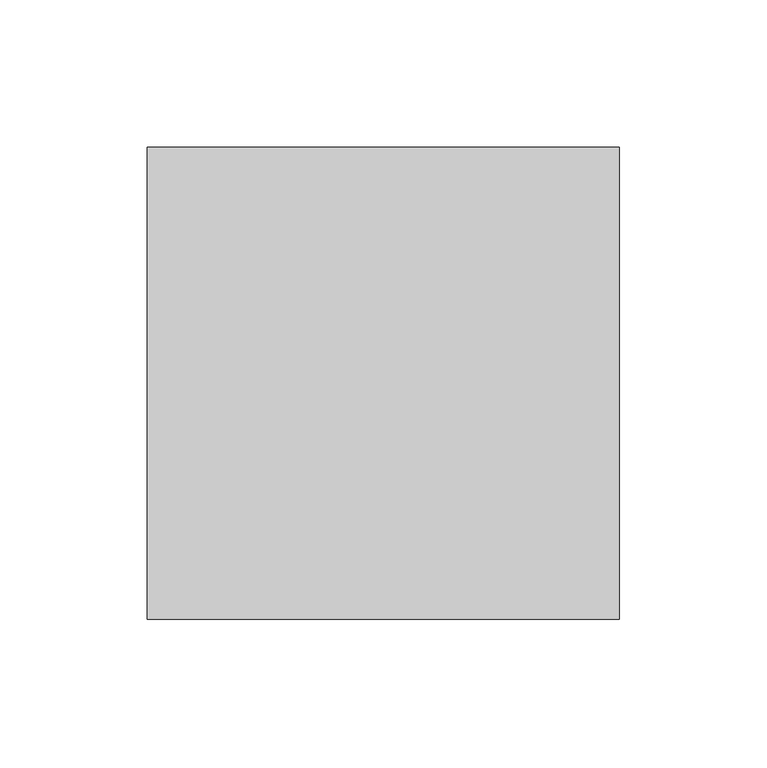
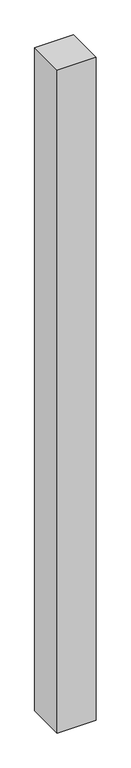
"""IFC4 building model written with IfcOpenShell, lengths in millimetres: column geometry, 0_3d."""

import ifcopenshell
import ifcopenshell.guid

model = None  # the IFC model being written
_history = None  # IfcOwnerHistory: only IFC2X3 demands one
_inside = {}  # id of a spatial element -> (the spatial element, [elements in it])
_under = {}  # id of a project, library or spatial element -> (it, [spatial elements below it])
_declared = {}  # id of a project -> (the project, [libraries it declares])
_typed = {}  # id of a type object -> (the type object, [elements of that type])
_made_of = {}  # id of a material, layer set ... -> (it, [elements and type objects made of it])


def new_model(schema):
    """Start an empty IFC model of exactly this schema.

    Asked for "IFC4X3", IfcOpenShell would pick the latest addendum, in which some entities
    have other attributes; the version numbers below select the first issue.
    IFC2X3 requires an IfcOwnerHistory on every rooted entity: one is made here for all.
    """
    global model, _history
    if schema == "IFC4X3":
        model = ifcopenshell.file(schema_version=(4, 3, 0, 0))
    else:
        model = ifcopenshell.file(schema=schema)
    _inside.clear()
    _under.clear()
    _declared.clear()
    _typed.clear()
    _made_of.clear()
    _history = None
    if model.schema == "IFC2X3":
        org = make("IfcOrganization", Name="unknown")
        user = make(
            "IfcPersonAndOrganization",
            ThePerson=make("IfcPerson", FamilyName="unknown"),
            TheOrganization=org,
        )
        app = make(
            "IfcApplication",
            ApplicationDeveloper=org,
            Version="unknown",
            ApplicationFullName="unknown",
            ApplicationIdentifier="unknown",
        )
        _history = make(
            "IfcOwnerHistory",
            OwningUser=user,
            OwningApplication=app,
            ChangeAction="ADDED",
            CreationDate=0,
        )
    return model


def make(cls, **values):
    """One entity of the class cls with the attributes given. An attribute that is None is left unset."""
    return model.create_entity(
        cls, **{name: value for name, value in values.items() if value is not None}
    )


def rooted(cls, **values):
    """An entity with a GlobalId (a new one), such as an element, a storey or a relation."""
    return make(cls, GlobalId=ifcopenshell.guid.new(), OwnerHistory=_history, **values)


def si_unit(unit_type, name, prefix=None):
    """IfcSIUnit, for example si_unit("LENGTHUNIT", "METRE", prefix="MILLI")."""
    return make("IfcSIUnit", UnitType=unit_type, Prefix=prefix, Name=name)


def assignment(units):
    """IfcUnitAssignment: the units of a project."""
    return None if units is None else make("IfcUnitAssignment", Units=units)


def point(xyz):
    """IfcCartesianPoint."""
    return None if xyz is None else make("IfcCartesianPoint", Coordinates=xyz)


def direction(xyz):
    """IfcDirection."""
    return None if xyz is None else make("IfcDirection", DirectionRatios=xyz)


def frame(location, z_axis=None, x_axis=None):
    """IfcAxis2Placement3D, a coordinate frame: its origin and axes. An axis left out is left unset."""
    return make(
        "IfcAxis2Placement3D",
        Location=point(location),
        Axis=direction(z_axis),
        RefDirection=direction(x_axis),
    )


def origin():
    """The frame at (0, 0, 0) with its axes left unset."""
    return frame((0.0, 0.0, 0.0))


def origin_with_axes():
    """The frame at (0, 0, 0) with the z axis (0, 0, 1) and the x axis (1, 0, 0) written out."""
    return frame((0.0, 0.0, 0.0), z_axis=(0.0, 0.0, 1.0), x_axis=(1.0, 0.0, 0.0))


def place(relative_to, where):
    """IfcLocalPlacement: puts the frame where relative to a parent placement (None: the world)."""
    return make(
        "IfcLocalPlacement", PlacementRelTo=relative_to, RelativePlacement=where
    )


def context(
    kind, dimensions, precision=None, world=None, true_north=None, identifier=None
):
    """IfcGeometricRepresentationContext, for example the 3D "Model" context."""
    return make(
        "IfcGeometricRepresentationContext",
        ContextIdentifier=identifier,
        ContextType=kind,
        CoordinateSpaceDimension=dimensions,
        Precision=precision,
        WorldCoordinateSystem=world,
        TrueNorth=true_north,
    )


def project(units=None, contexts=None):
    """IfcProject with its units and contexts."""
    return rooted(
        "IfcProject",
        Name="project",
        RepresentationContexts=contexts,
        UnitsInContext=assignment(units),
    )


def spatial(cls, under=None, at=None, **own):
    """A site, building, storey or space (cls), placed at a placement, below another one or the project."""
    s = rooted(cls, ObjectPlacement=at, **own)
    if under is not None:
        _under.setdefault(under.id(), (under, []))[1].append(s)
    return s


def polyline(points):
    """IfcPolyline through the points."""
    return make("IfcPolyline", Points=[point(p) for p in points])


def outline(outer, holes=None, kind="AREA"):
    """IfcArbitraryClosedProfileDef: a profile drawn as a closed curve; with holes, ...WithVoids."""
    if holes is None:
        return make("IfcArbitraryClosedProfileDef", ProfileType=kind, OuterCurve=outer)
    return make(
        "IfcArbitraryProfileDefWithVoids",
        ProfileType=kind,
        OuterCurve=outer,
        InnerCurves=holes,
    )


def extrude(swept, where, along, depth):
    """IfcExtrudedAreaSolid: the profile swept, set in the frame where, extruded along a direction by depth."""
    return make(
        "IfcExtrudedAreaSolid",
        SweptArea=swept,
        Position=where,
        ExtrudedDirection=direction(along),
        Depth=depth,
    )


def shape(context_of_items, identifier, shape_type, items):
    """IfcShapeRepresentation: the items that make up one representation, for example the "Body"."""
    return make(
        "IfcShapeRepresentation",
        ContextOfItems=context_of_items,
        RepresentationIdentifier=identifier,
        RepresentationType=shape_type,
        Items=items,
    )


def source(mapping_origin, context_of_items, identifier, shape_type, items):
    """IfcRepresentationMap: a shape defined once, which mapped items show again and again."""
    return make(
        "IfcRepresentationMap",
        MappingOrigin=mapping_origin,
        MappedRepresentation=shape(context_of_items, identifier, shape_type, items),
    )


def transform(
    local_origin,
    x_axis=None,
    y_axis=None,
    z_axis=None,
    scale=None,
    scale2=None,
    scale3=None,
    uniform=True,
):
    """IfcCartesianTransformationOperator3D, or its non-uniform kind. x_axis, y_axis, z_axis: its Axis1, 2, 3."""
    if uniform:
        return make(
            "IfcCartesianTransformationOperator3D",
            Axis1=direction(x_axis),
            Axis2=direction(y_axis),
            LocalOrigin=point(local_origin),
            Scale=scale,
            Axis3=direction(z_axis),
        )
    return make(
        "IfcCartesianTransformationOperator3DnonUniform",
        Axis1=direction(x_axis),
        Axis2=direction(y_axis),
        LocalOrigin=point(local_origin),
        Scale=scale,
        Axis3=direction(z_axis),
        Scale2=scale2,
        Scale3=scale3,
    )


def mapped(mapping_source, mapping_target):
    """IfcMappedItem: shows the shape of a source again, moved by a transform."""
    return make(
        "IfcMappedItem", MappingSource=mapping_source, MappingTarget=mapping_target
    )


def made_of(thing, what):
    """Note that an element or type object is made of a material, layer set ...; save() writes the relation."""
    if what is not None:
        _made_of.setdefault(what.id(), (what, []))[1].append(thing)
    return thing


def element(
    cls,
    number,
    at=None,
    inside=None,
    cuts=None,
    type_object=None,
    material=None,
    context=None,
    identifier="Body",
    shape_type=None,
    held_by="IfcProductDefinitionShape",
    body=None,
    shapes=None,
    **own,
):
    """One element of the class cls, such as IfcWall. Its Tag is "e" and its number.

    at: its placement. inside: the storey or other place that contains it. cuts: it is an
    opening in that element (IfcRelVoidsElement). A single representation is given by context,
    identifier, shape_type and body (its items); several are given by shapes. held_by: the class
    of the entity that holds the representations. save() writes the other relations.
    """
    e = rooted(cls, Tag="e%d" % number, ObjectPlacement=at, **own)
    if body is not None:
        shapes = [shape(context, identifier, shape_type, body)]
    if shapes is not None:
        e.Representation = make(held_by, Representations=shapes)
    if inside is not None:
        _inside.setdefault(inside.id(), (inside, []))[1].append(e)
    if cuts is not None:
        rooted(
            "IfcRelVoidsElement", RelatingBuildingElement=cuts, RelatedOpeningElement=e
        )
    if type_object is not None:
        _typed.setdefault(type_object.id(), (type_object, []))[1].append(e)
    return made_of(e, material)


def aggregate(whole, parts):
    """IfcRelAggregates: a whole, such as a stair, and the parts it consists of."""
    return rooted("IfcRelAggregates", RelatingObject=whole, RelatedObjects=parts)


def save(model, path):
    """Write the relations noted so far, then the file.

    IfcRelAggregates (storeys below a building ...), IfcRelContainedInSpatialStructure (elements
    in a storey), IfcRelDefinesByType, IfcRelAssociatesMaterial and IfcRelDeclares: one each for
    every whole, place, type object, material and project.
    """
    for whole, parts in _under.values():
        aggregate(whole, parts)
    for where, things in _inside.values():
        rooted(
            "IfcRelContainedInSpatialStructure",
            RelatedElements=things,
            RelatingStructure=where,
        )
    for kind, things in _typed.values():
        rooted("IfcRelDefinesByType", RelatedObjects=things, RelatingType=kind)
    for what, things in _made_of.values():
        rooted("IfcRelAssociatesMaterial", RelatedObjects=things, RelatingMaterial=what)
    for by, libraries in _declared.values():
        rooted("IfcRelDeclares", RelatingContext=by, RelatedDefinitions=libraries)
    model.write(path)


def column_a3602641(model_context):
    return source(origin(), model_context, "Body", "SweptSolid", [
        extrude(outline(polyline([(160.0, 160.0), (160.0, 0.0), (0.0, 0.0), (0.0, 160.0), (160.0, 160.0)])), origin_with_axes(), (0.0, 0.0, 1.0), 2880.0),
    ])


if __name__ == "__main__":
    model = new_model("IFC4")
    model_context = context("Model", 3, world=origin())
    ifc_project = project(units=[si_unit("LENGTHUNIT", "METRE", prefix="MILLI")], contexts=[model_context])
    site = spatial("IfcSite", under=ifc_project)
    building = spatial("IfcBuilding", under=site)
    placement = place(None, origin())
    column_shape = column_a3602641(model_context)
    element("IfcColumn", 1, ObjectType="0_3d", at=placement, inside=building, context=model_context, shape_type="MappedRepresentation", body=[
        mapped(column_shape, transform((0.0, 0.0, 0.0), x_axis=(1.0, 0.0, 0.0), y_axis=(0.0, 1.0, 0.0), z_axis=(0.0, 0.0, 1.0))),
    ])
    save(model, "model.ifc")

# Revit data of these elements
# Element 1 (IfcColumn, "0_3d")
#   Materials on its faces: "material wardrobe b 1"
# Materials
#   "material wardrobe b 1": class "Unassigned", colour RGB 128 128 128, transparency 0
